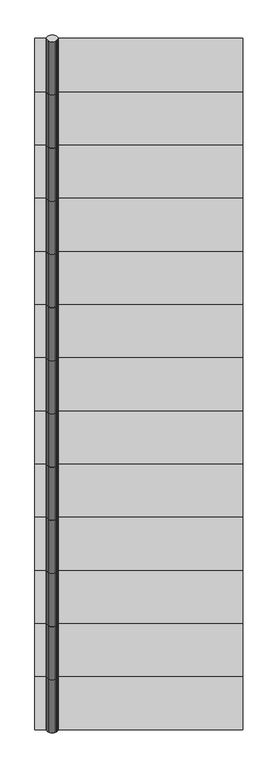
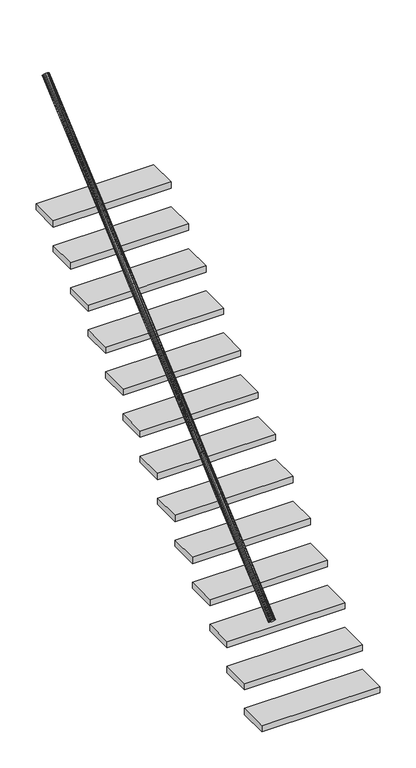
"""IFC4 building model written with IfcOpenShell, lengths in millimetres: stair geometry, 0_3d."""

from ifc_helpers import new_model, si_unit, frame, origin, origin_with_axes, place, context, project, spatial, polyline, outline, extrude, source, transform, mapped, element, save


def stair_fb9413d2(model_context):
    return source(origin(), model_context, "Body", "SweptSolid", [
        extrude(outline(polyline([(0.0, 705.003504), (0.0, 935.003504), (900.0, 935.003504), (900.0, 705.003504), (0.0, 705.003504)])), frame((0.0, 0.0, 600.0), z_axis=(0.0, 0.0, 1.0), x_axis=(1.0, 0.0, 0.0)), (0.0, 0.0, 1.0), 50.0),
        extrude(outline(polyline([(0.0, 245.003504), (0.0, 475.003504), (900.0, 475.003504), (900.0, 245.003504), (0.0, 245.003504)])), frame((0.0, 0.0, 200.0), z_axis=(0.0, 0.0, 1.0), x_axis=(1.0, 0.0, 0.0)), (0.0, 0.0, 1.0), 50.0),
        extrude(outline(polyline([(0.0, 475.003504), (0.0, 705.003504), (900.0, 705.003504), (900.0, 475.003504), (0.0, 475.003504)])), frame((0.0, 0.0, 400.0), z_axis=(0.0, 0.0, 1.0), x_axis=(1.0, 0.0, 0.0)), (0.0, 0.0, 1.0), 50.0),
        extrude(outline(polyline([(1.2235871, -7.065663), (0.0, 0.0), (1.2235871, 7.0656631), (4.7745751, 13.4396898), (10.3053687, 18.498146), (17.2745751, 21.7458748), (25.0, 22.864966), (32.7254249, 21.7458748), (39.6946313, 18.498146), (45.2254249, 13.4396898), (48.7764129, 7.0656631), (50.0, 0.0), (48.7764129, -7.065663), (45.2254249, -13.4396897), (39.6946313, -18.4981459), (32.7254249, -21.7458748), (25.0, -22.8649659), (17.2745751, -21.7458748), (10.3053687, -18.4981459), (4.7745751, -13.4396897), (1.2235871, -7.065663)])), frame((100.0, 705.003504, 1469.5592366), z_axis=(0.0, 0.754605522163452, 0.6561787149248474), x_axis=(-1.0, 0.0, 0.0)), (0.0, 0.0, 1.0), 304.7950131),
        extrude(outline(polyline([(1.2235871, -7.065663), (0.0, 0.0), (1.2235871, 7.0656631), (4.7745751, 13.4396898), (10.3053687, 18.498146), (17.2745751, 21.7458748), (25.0, 22.864966), (32.7254249, 21.7458748), (39.6946313, 18.498146), (45.2254249, 13.4396898), (48.7764129, 7.0656631), (50.0, 0.0), (48.7764129, -7.065663), (45.2254249, -13.4396897), (39.6946313, -18.4981459), (32.7254249, -21.7458748), (25.0, -22.8649659), (17.2745751, -21.7458748), (10.3053687, -18.4981459), (4.7745751, -13.4396897), (1.2235871, -7.065663)])), frame((100.0, 245.003504, 1069.5592366), z_axis=(0.0, 0.7546055221634516, 0.6561787149248478), x_axis=(-1.0, 0.0, 0.0)), (0.0, 0.0, 1.0), 304.7950131),
        extrude(outline(polyline([(1.2235871, -7.065663), (0.0, 0.0), (1.2235871, 7.0656631), (4.7745751, 13.4396898), (10.3053687, 18.498146), (17.2745751, 21.7458748), (25.0, 22.864966), (32.7254249, 21.7458748), (39.6946313, 18.498146), (45.2254249, 13.4396898), (48.7764129, 7.0656631), (50.0, 0.0), (48.7764129, -7.065663), (45.2254249, -13.4396897), (39.6946313, -18.4981459), (32.7254249, -21.7458748), (25.0, -22.8649659), (17.2745751, -21.7458748), (10.3053687, -18.4981459), (4.7745751, -13.4396897), (1.2235871, -7.065663)])), frame((100.0, 15.003504, 869.5592366), z_axis=(0.0, 0.7546055221634684, 0.6561787149248285), x_axis=(-1.0, 0.0, 0.0)), (0.0, 0.0, 1.0), 304.7950131),
        extrude(outline(polyline([(0.0, 2775.003504), (0.0, 3005.003504), (900.0, 3005.003504), (900.0, 2775.003504), (0.0, 2775.003504)])), frame((0.0, 0.0, 2400.0), z_axis=(0.0, 0.0, 1.0), x_axis=(1.0, 0.0, 0.0)), (0.0, 0.0, 1.0), 50.0),
        extrude(outline(polyline([(1.2235871, -7.065663), (0.0, 0.0), (1.2235871, 7.0656631), (4.7745751, 13.4396898), (10.3053687, 18.498146), (17.2745751, 21.7458748), (25.0, 22.864966), (32.7254249, 21.7458748), (39.6946313, 18.498146), (45.2254249, 13.4396898), (48.7764129, 7.0656631), (50.0, 0.0), (48.7764129, -7.065663), (45.2254249, -13.4396897), (39.6946313, -18.4981459), (32.7254249, -21.7458748), (25.0, -22.8649659), (17.2745751, -21.7458748), (10.3053687, -18.4981459), (4.7745751, -13.4396897), (1.2235871, -7.065663)])), frame((100.0, 475.003504, 1269.5592366), z_axis=(0.0, 0.7546055221634538, 0.6561787149248451), x_axis=(-1.0, 0.0, 0.0)), (0.0, 0.0, 1.0), 304.7950131),
        extrude(outline(polyline([(0.0, 1625.003504), (0.0, 1855.003504), (900.0, 1855.003504), (900.0, 1625.003504), (0.0, 1625.003504)])), frame((0.0, 0.0, 1400.0), z_axis=(0.0, 0.0, 1.0), x_axis=(1.0, 0.0, 0.0)), (0.0, 0.0, 1.0), 50.0),
        extrude(outline(polyline([(1.2235871, -7.065663), (0.0, 0.0), (1.2235871, 7.0656631), (4.7745751, 13.4396898), (10.3053687, 18.498146), (17.2745751, 21.7458748), (25.0, 22.864966), (32.7254249, 21.7458748), (39.6946313, 18.498146), (45.2254249, 13.4396898), (48.7764129, 7.0656631), (50.0, 0.0), (48.7764129, -7.065663), (45.2254249, -13.4396897), (39.6946313, -18.4981459), (32.7254249, -21.7458748), (25.0, -22.8649659), (17.2745751, -21.7458748), (10.3053687, -18.4981459), (4.7745751, -13.4396897), (1.2235871, -7.065663)])), frame((100.0, 2545.003504, 3069.5592366), z_axis=(0.0, 0.7546055221634004, 0.6561787149249066), x_axis=(-1.0, 0.0, 0.0)), (0.0, 0.0, 1.0), 304.7950131),
        extrude(outline(polyline([(1.2235871, -7.065663), (0.0, 0.0), (1.2235871, 7.0656631), (4.7745751, 13.4396898), (10.3053687, 18.498146), (17.2745751, 21.7458748), (25.0, 22.864966), (32.7254249, 21.7458748), (39.6946313, 18.498146), (45.2254249, 13.4396898), (48.7764129, 7.0656631), (50.0, 0.0), (48.7764129, -7.065663), (45.2254249, -13.4396897), (39.6946313, -18.4981459), (32.7254249, -21.7458748), (25.0, -22.8649659), (17.2745751, -21.7458748), (10.3053687, -18.4981459), (4.7745751, -13.4396897), (1.2235871, -7.065663)])), frame((100.0, 1165.003504, 1869.5592366), z_axis=(0.0, 0.7546055221634032, 0.6561787149249034), x_axis=(-1.0, 0.0, 0.0)), (0.0, 0.0, 1.0), 304.7950131),
        extrude(outline(polyline([(1.2235871, -7.065663), (0.0, 0.0), (1.2235871, 7.0656631), (4.7745751, 13.4396898), (10.3053687, 18.498146), (17.2745751, 21.7458748), (25.0, 22.864966), (32.7254249, 21.7458748), (39.6946313, 18.498146), (45.2254249, 13.4396898), (48.7764129, 7.0656631), (50.0, 0.0), (48.7764129, -7.065663), (45.2254249, -13.4396897), (39.6946313, -18.4981459), (32.7254249, -21.7458748), (25.0, -22.8649659), (17.2745751, -21.7458748), (10.3053687, -18.4981459), (4.7745751, -13.4396897), (1.2235871, -7.065663)])), frame((100.0, 1625.003504, 2269.5592366), z_axis=(0.0, 0.7546055221634113, 0.6561787149248941), x_axis=(-1.0, 0.0, 0.0)), (0.0, 0.0, 1.0), 304.7950131),
        extrude(outline(polyline([(0.0, 15.003504), (0.0, 245.003504), (900.0, 245.003504), (900.0, 15.003504), (0.0, 15.003504)])), origin_with_axes(), (0.0, 0.0, 1.0), 50.0),
        extrude(outline(polyline([(0.0, 2545.003504), (0.0, 2775.003504), (900.0, 2775.003504), (900.0, 2545.003504), (0.0, 2545.003504)])), frame((0.0, 0.0, 2200.0), z_axis=(0.0, 0.0, 1.0), x_axis=(1.0, 0.0, 0.0)), (0.0, 0.0, 1.0), 50.0),
        extrude(outline(polyline([(0.0, 1165.003504), (0.0, 1395.003504), (900.0, 1395.003504), (900.0, 1165.003504), (0.0, 1165.003504)])), frame((0.0, 0.0, 1000.0), z_axis=(0.0, 0.0, 1.0), x_axis=(1.0, 0.0, 0.0)), (0.0, 0.0, 1.0), 50.0),
        extrude(outline(polyline([(1.2235871, -7.065663), (0.0, 0.0), (1.2235871, 7.0656631), (4.7745751, 13.4396898), (10.3053687, 18.498146), (17.2745751, 21.7458748), (25.0, 22.864966), (32.7254249, 21.7458748), (39.6946313, 18.498146), (45.2254249, 13.4396898), (48.7764129, 7.0656631), (50.0, 0.0), (48.7764129, -7.065663), (45.2254249, -13.4396897), (39.6946313, -18.4981459), (32.7254249, -21.7458748), (25.0, -22.8649659), (17.2745751, -21.7458748), (10.3053687, -18.4981459), (4.7745751, -13.4396897), (1.2235871, -7.065663)])), frame((100.0, 2775.003504, 3269.5592366), z_axis=(0.0, 0.7546055221633948, 0.656178714924913), x_axis=(-1.0, 0.0, 0.0)), (0.0, 0.0, 1.0), 304.7950131),
        extrude(outline(polyline([(1.2235871, -7.065663), (0.0, 0.0), (1.2235871, 7.0656631), (4.7745751, 13.4396898), (10.3053687, 18.498146), (17.2745751, 21.7458748), (25.0, 22.864966), (32.7254249, 21.7458748), (39.6946313, 18.498146), (45.2254249, 13.4396898), (48.7764129, 7.0656631), (50.0, 0.0), (48.7764129, -7.065663), (45.2254249, -13.4396897), (39.6946313, -18.4981459), (32.7254249, -21.7458748), (25.0, -22.8649659), (17.2745751, -21.7458748), (10.3053687, -18.4981459), (4.7745751, -13.4396897), (1.2235871, -7.065663)])), frame((100.0, 2315.003504, 2869.5592366), z_axis=(0.0, 0.7546055221634095, 0.6561787149248961), x_axis=(-1.0, 0.0, 0.0)), (0.0, 0.0, 1.0), 304.7950131),
        extrude(outline(polyline([(0.0, 1395.003504), (0.0, 1625.003504), (900.0, 1625.003504), (900.0, 1395.003504), (0.0, 1395.003504)])), frame((0.0, 0.0, 1200.0), z_axis=(0.0, 0.0, 1.0), x_axis=(1.0, 0.0, 0.0)), (0.0, 0.0, 1.0), 50.0),
        extrude(outline(polyline([(0.0, 935.003504), (0.0, 1165.003504), (900.0, 1165.003504), (900.0, 935.003504), (0.0, 935.003504)])), frame((0.0, 0.0, 800.0), z_axis=(0.0, 0.0, 1.0), x_axis=(1.0, 0.0, 0.0)), (0.0, 0.0, 1.0), 50.0),
        extrude(outline(polyline([(0.0, 2315.003504), (0.0, 2545.003504), (900.0, 2545.003504), (900.0, 2315.003504), (0.0, 2315.003504)])), frame((0.0, 0.0, 2000.0), z_axis=(0.0, 0.0, 1.0), x_axis=(1.0, 0.0, 0.0)), (0.0, 0.0, 1.0), 50.0),
        extrude(outline(polyline([(1.2235871, -7.065663), (0.0, 0.0), (1.2235871, 7.0656631), (4.7745751, 13.4396898), (10.3053687, 18.498146), (17.2745751, 21.7458748), (25.0, 22.864966), (32.7254249, 21.7458748), (39.6946313, 18.498146), (45.2254249, 13.4396898), (48.7764129, 7.0656631), (50.0, 0.0), (48.7764129, -7.065663), (45.2254249, -13.4396897), (39.6946313, -18.4981459), (32.7254249, -21.7458748), (25.0, -22.8649659), (17.2745751, -21.7458748), (10.3053687, -18.4981459), (4.7745751, -13.4396897), (1.2235871, -7.065663)])), frame((100.0, 935.003504, 1669.5592366), z_axis=(0.0, 0.754605522163451, 0.6561787149248486), x_axis=(-1.0, 0.0, 0.0)), (0.0, 0.0, 1.0), 304.7950131),
        extrude(outline(polyline([(0.0, 2085.003504), (0.0, 2315.003504), (900.0, 2315.003504), (900.0, 2085.003504), (0.0, 2085.003504)])), frame((0.0, 0.0, 1800.0), z_axis=(0.0, 0.0, 1.0), x_axis=(1.0, 0.0, 0.0)), (0.0, 0.0, 1.0), 50.0),
        extrude(outline(polyline([(1.2235871, -7.065663), (0.0, 0.0), (1.2235871, 7.0656631), (4.7745751, 13.4396898), (10.3053687, 18.498146), (17.2745751, 21.7458748), (25.0, 22.864966), (32.7254249, 21.7458748), (39.6946313, 18.498146), (45.2254249, 13.4396898), (48.7764129, 7.0656631), (50.0, 0.0), (48.7764129, -7.065663), (45.2254249, -13.4396897), (39.6946313, -18.4981459), (32.7254249, -21.7458748), (25.0, -22.8649659), (17.2745751, -21.7458748), (10.3053687, -18.4981459), (4.7745751, -13.4396897), (1.2235871, -7.065663)])), frame((100.0, 1855.003504, 2469.5592366), z_axis=(0.0, 0.7546055221634099, 0.6561787149248958), x_axis=(-1.0, 0.0, 0.0)), (0.0, 0.0, 1.0), 304.7950131),
        extrude(outline(polyline([(1.2235871, -7.065663), (0.0, 0.0), (1.2235871, 7.0656631), (4.7745751, 13.4396898), (10.3053687, 18.498146), (17.2745751, 21.7458748), (25.0, 22.864966), (32.7254249, 21.7458748), (39.6946313, 18.498146), (45.2254249, 13.4396898), (48.7764129, 7.0656631), (50.0, 0.0), (48.7764129, -7.065663), (45.2254249, -13.4396897), (39.6946313, -18.4981459), (32.7254249, -21.7458748), (25.0, -22.8649659), (17.2745751, -21.7458748), (10.3053687, -18.4981459), (4.7745751, -13.4396897), (1.2235871, -7.065663)])), frame((100.0, 1395.003504, 2069.5592366), z_axis=(0.0, 0.7546055221634036, 0.6561787149249029), x_axis=(-1.0, 0.0, 0.0)), (0.0, 0.0, 1.0), 304.7950131),
        extrude(outline(polyline([(0.0, 1855.003504), (0.0, 2085.003504), (900.0, 2085.003504), (900.0, 1855.003504), (0.0, 1855.003504)])), frame((0.0, 0.0, 1600.0), z_axis=(0.0, 0.0, 1.0), x_axis=(1.0, 0.0, 0.0)), (0.0, 0.0, 1.0), 50.0),
        extrude(outline(polyline([(1.2235871, -7.065663), (0.0, 0.0), (1.2235871, 7.0656631), (4.7745751, 13.4396898), (10.3053687, 18.498146), (17.2745751, 21.7458748), (25.0, 22.864966), (32.7254249, 21.7458748), (39.6946313, 18.498146), (45.2254249, 13.4396898), (48.7764129, 7.0656631), (50.0, 0.0), (48.7764129, -7.065663), (45.2254249, -13.4396897), (39.6946313, -18.4981459), (32.7254249, -21.7458748), (25.0, -22.8649659), (17.2745751, -21.7458748), (10.3053687, -18.4981459), (4.7745751, -13.4396897), (1.2235871, -7.065663)])), frame((100.0, 2085.003504, 2669.5592366), z_axis=(0.0, 0.7546055221634052, 0.6561787149249011), x_axis=(-1.0, 0.0, 0.0)), (0.0, 0.0, 1.0), 304.7950131),
    ])


if __name__ == "__main__":
    model = new_model("IFC4")
    model_context = context("Model", 3, world=origin())
    ifc_project = project(units=[si_unit("LENGTHUNIT", "METRE", prefix="MILLI")], contexts=[model_context])
    site = spatial("IfcSite", under=ifc_project)
    building = spatial("IfcBuilding", under=site)
    placement = place(None, origin())
    stair_shape = stair_fb9413d2(model_context)
    element("IfcStair", 1, ObjectType="0_3d", at=placement, inside=building, context=model_context, shape_type="MappedRepresentation", body=[
        mapped(stair_shape, transform((0.0, 0.0, 0.0), x_axis=(1.0, 0.0, 0.0), y_axis=(0.0, 1.0, 0.0), z_axis=(0.0, 0.0, 1.0))),
    ])
    save(model, "model.ifc")

# Revit data of these elements
# Element 1 (IfcStair, "0_3d")
#   Materials on its faces: "*1", "weiss"
# Materials
#   "*1": class "Unassigned", colour RGB 175 175 175, transparency 0
#   "weiss": class "Unassigned", colour RGB 255 255 255, transparency 0
